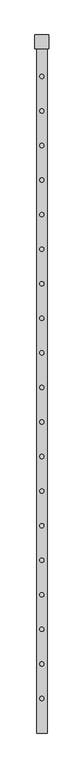
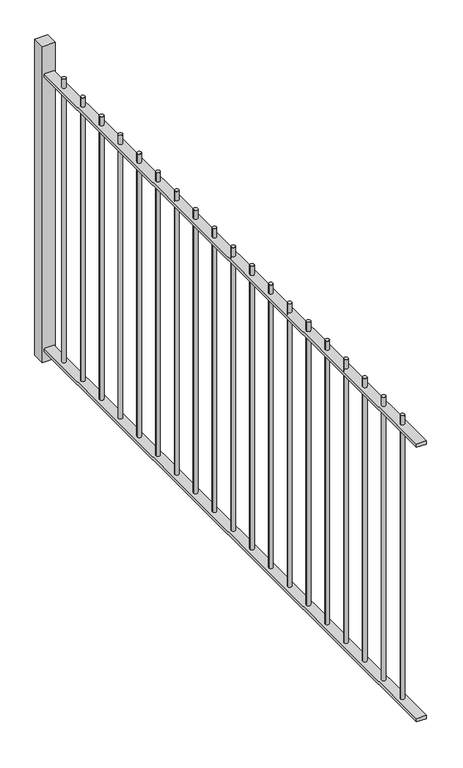
"""IFC4 building model written with IfcOpenShell, lengths in millimetres: railing geometry."""

from ifc_helpers import new_model, si_unit, point, frame, frame_2d, origin, place, context, project, spatial, polyline, circle_curve, trimmed, segment, composite_curve, outline, extrude, source, transform, mapped, element, save


def railing_93278f43(model_context):
    return source(origin(), model_context, "Body", "SweptSolid", [
        extrude(outline(polyline([(-6549.419961, -691.1119119), (-6489.419961, -691.1119119), (-6489.419961, -4691.1119119), (-6549.419961, -4691.1119119), (-6549.419961, -691.1119119)])), frame((0.0, 0.0, -30.0), z_axis=(0.0, 0.0, 1.0), x_axis=(1.0, 0.0, 0.0)), (0.0, 0.0, 1.0), 20.0),
        extrude(outline(polyline([(-6549.419961, -691.1119119), (-6489.419961, -691.1119119), (-6489.419961, -4691.1119119), (-6549.419961, -4691.1119119), (-6549.419961, -691.1119119)])), frame((0.0, 0.0, 1750.0), z_axis=(0.0, 0.0, 1.0), x_axis=(1.0, 0.0, 0.0)), (0.0, 0.0, 1.0), 20.0),
        extrude(outline(composite_curve([segment(trimmed(circle_curve(frame_2d((-6519.419961, -4491.1119119)), 12.5), [point((-6531.919961, -4491.1119119))], [point((-6506.919961, -4491.1119119))], False, "CARTESIAN"), True, "CONTINUOUS"), segment(trimmed(circle_curve(frame_2d((-6519.419961, -4491.1119119)), 12.5), [point((-6506.919961, -4491.1119119))], [point((-6531.919961, -4491.1119119))], False, "CARTESIAN"), True, "CONTINUOUS")], self_intersect=False)), frame((0.0, 0.0, -10.0), z_axis=(0.0, 0.0, 1.0), x_axis=(1.0, 0.0, 0.0)), (0.0, 0.0, 1.0), 1840.0),
        extrude(outline(composite_curve([segment(trimmed(circle_curve(frame_2d((-6519.419961, -4291.1119119)), 12.5), [point((-6531.919961, -4291.1119119))], [point((-6506.919961, -4291.1119119))], False, "CARTESIAN"), True, "CONTINUOUS"), segment(trimmed(circle_curve(frame_2d((-6519.419961, -4291.1119119)), 12.5), [point((-6506.919961, -4291.1119119))], [point((-6531.919961, -4291.1119119))], False, "CARTESIAN"), True, "CONTINUOUS")], self_intersect=False)), frame((0.0, 0.0, -10.0), z_axis=(0.0, 0.0, 1.0), x_axis=(1.0, 0.0, 0.0)), (0.0, 0.0, 1.0), 1840.0),
        extrude(outline(composite_curve([segment(trimmed(circle_curve(frame_2d((-6519.419961, -4091.1119119)), 12.5), [point((-6531.919961, -4091.1119119))], [point((-6506.919961, -4091.1119119))], False, "CARTESIAN"), True, "CONTINUOUS"), segment(trimmed(circle_curve(frame_2d((-6519.419961, -4091.1119119)), 12.5), [point((-6506.919961, -4091.1119119))], [point((-6531.919961, -4091.1119119))], False, "CARTESIAN"), True, "CONTINUOUS")], self_intersect=False)), frame((0.0, 0.0, -10.0), z_axis=(0.0, 0.0, 1.0), x_axis=(1.0, 0.0, 0.0)), (0.0, 0.0, 1.0), 1840.0),
        extrude(outline(composite_curve([segment(trimmed(circle_curve(frame_2d((-6519.419961, -3891.1119119)), 12.5), [point((-6531.919961, -3891.1119119))], [point((-6506.919961, -3891.1119119))], False, "CARTESIAN"), True, "CONTINUOUS"), segment(trimmed(circle_curve(frame_2d((-6519.419961, -3891.1119119)), 12.5), [point((-6506.919961, -3891.1119119))], [point((-6531.919961, -3891.1119119))], False, "CARTESIAN"), True, "CONTINUOUS")], self_intersect=False)), frame((0.0, 0.0, -10.0), z_axis=(0.0, 0.0, 1.0), x_axis=(1.0, 0.0, 0.0)), (0.0, 0.0, 1.0), 1840.0),
        extrude(outline(composite_curve([segment(trimmed(circle_curve(frame_2d((-6519.419961, -3691.1119119)), 12.5), [point((-6531.919961, -3691.1119119))], [point((-6506.919961, -3691.1119119))], False, "CARTESIAN"), True, "CONTINUOUS"), segment(trimmed(circle_curve(frame_2d((-6519.419961, -3691.1119119)), 12.5), [point((-6506.919961, -3691.1119119))], [point((-6531.919961, -3691.1119119))], False, "CARTESIAN"), True, "CONTINUOUS")], self_intersect=False)), frame((0.0, 0.0, -10.0), z_axis=(0.0, 0.0, 1.0), x_axis=(1.0, 0.0, 0.0)), (0.0, 0.0, 1.0), 1840.0),
        extrude(outline(composite_curve([segment(trimmed(circle_curve(frame_2d((-6519.419961, -3491.1119119)), 12.5), [point((-6531.919961, -3491.1119119))], [point((-6506.919961, -3491.1119119))], False, "CARTESIAN"), True, "CONTINUOUS"), segment(trimmed(circle_curve(frame_2d((-6519.419961, -3491.1119119)), 12.5), [point((-6506.919961, -3491.1119119))], [point((-6531.919961, -3491.1119119))], False, "CARTESIAN"), True, "CONTINUOUS")], self_intersect=False)), frame((0.0, 0.0, -10.0), z_axis=(0.0, 0.0, 1.0), x_axis=(1.0, 0.0, 0.0)), (0.0, 0.0, 1.0), 1840.0),
        extrude(outline(composite_curve([segment(trimmed(circle_curve(frame_2d((-6519.419961, -3291.1119119)), 12.5), [point((-6531.919961, -3291.1119119))], [point((-6506.919961, -3291.1119119))], False, "CARTESIAN"), True, "CONTINUOUS"), segment(trimmed(circle_curve(frame_2d((-6519.419961, -3291.1119119)), 12.5), [point((-6506.919961, -3291.1119119))], [point((-6531.919961, -3291.1119119))], False, "CARTESIAN"), True, "CONTINUOUS")], self_intersect=False)), frame((0.0, 0.0, -10.0), z_axis=(0.0, 0.0, 1.0), x_axis=(1.0, 0.0, 0.0)), (0.0, 0.0, 1.0), 1840.0),
        extrude(outline(composite_curve([segment(trimmed(circle_curve(frame_2d((-6519.419961, -3091.1119119)), 12.5), [point((-6531.919961, -3091.1119119))], [point((-6506.919961, -3091.1119119))], False, "CARTESIAN"), True, "CONTINUOUS"), segment(trimmed(circle_curve(frame_2d((-6519.419961, -3091.1119119)), 12.5), [point((-6506.919961, -3091.1119119))], [point((-6531.919961, -3091.1119119))], False, "CARTESIAN"), True, "CONTINUOUS")], self_intersect=False)), frame((0.0, 0.0, -10.0), z_axis=(0.0, 0.0, 1.0), x_axis=(1.0, 0.0, 0.0)), (0.0, 0.0, 1.0), 1840.0),
        extrude(outline(composite_curve([segment(trimmed(circle_curve(frame_2d((-6519.419961, -2891.1119119)), 12.5), [point((-6531.919961, -2891.1119119))], [point((-6506.919961, -2891.1119119))], False, "CARTESIAN"), True, "CONTINUOUS"), segment(trimmed(circle_curve(frame_2d((-6519.419961, -2891.1119119)), 12.5), [point((-6506.919961, -2891.1119119))], [point((-6531.919961, -2891.1119119))], False, "CARTESIAN"), True, "CONTINUOUS")], self_intersect=False)), frame((0.0, 0.0, -10.0), z_axis=(0.0, 0.0, 1.0), x_axis=(1.0, 0.0, 0.0)), (0.0, 0.0, 1.0), 1840.0),
        extrude(outline(composite_curve([segment(trimmed(circle_curve(frame_2d((-6519.419961, -2691.1119119)), 12.5), [point((-6531.919961, -2691.1119119))], [point((-6506.919961, -2691.1119119))], False, "CARTESIAN"), True, "CONTINUOUS"), segment(trimmed(circle_curve(frame_2d((-6519.419961, -2691.1119119)), 12.5), [point((-6506.919961, -2691.1119119))], [point((-6531.919961, -2691.1119119))], False, "CARTESIAN"), True, "CONTINUOUS")], self_intersect=False)), frame((0.0, 0.0, -10.0), z_axis=(0.0, 0.0, 1.0), x_axis=(1.0, 0.0, 0.0)), (0.0, 0.0, 1.0), 1840.0),
        extrude(outline(composite_curve([segment(trimmed(circle_curve(frame_2d((-6519.419961, -2491.1119119)), 12.5), [point((-6531.919961, -2491.1119119))], [point((-6506.919961, -2491.1119119))], False, "CARTESIAN"), True, "CONTINUOUS"), segment(trimmed(circle_curve(frame_2d((-6519.419961, -2491.1119119)), 12.5), [point((-6506.919961, -2491.1119119))], [point((-6531.919961, -2491.1119119))], False, "CARTESIAN"), True, "CONTINUOUS")], self_intersect=False)), frame((0.0, 0.0, -10.0), z_axis=(0.0, 0.0, 1.0), x_axis=(1.0, 0.0, 0.0)), (0.0, 0.0, 1.0), 1840.0),
        extrude(outline(composite_curve([segment(trimmed(circle_curve(frame_2d((-6519.419961, -2291.1119119)), 12.5), [point((-6531.919961, -2291.1119119))], [point((-6506.919961, -2291.1119119))], False, "CARTESIAN"), True, "CONTINUOUS"), segment(trimmed(circle_curve(frame_2d((-6519.419961, -2291.1119119)), 12.5), [point((-6506.919961, -2291.1119119))], [point((-6531.919961, -2291.1119119))], False, "CARTESIAN"), True, "CONTINUOUS")], self_intersect=False)), frame((0.0, 0.0, -10.0), z_axis=(0.0, 0.0, 1.0), x_axis=(1.0, 0.0, 0.0)), (0.0, 0.0, 1.0), 1840.0),
        extrude(outline(composite_curve([segment(trimmed(circle_curve(frame_2d((-6519.419961, -2091.1119119)), 12.5), [point((-6531.919961, -2091.1119119))], [point((-6506.919961, -2091.1119119))], False, "CARTESIAN"), True, "CONTINUOUS"), segment(trimmed(circle_curve(frame_2d((-6519.419961, -2091.1119119)), 12.5), [point((-6506.919961, -2091.1119119))], [point((-6531.919961, -2091.1119119))], False, "CARTESIAN"), True, "CONTINUOUS")], self_intersect=False)), frame((0.0, 0.0, -10.0), z_axis=(0.0, 0.0, 1.0), x_axis=(1.0, 0.0, 0.0)), (0.0, 0.0, 1.0), 1840.0),
        extrude(outline(composite_curve([segment(trimmed(circle_curve(frame_2d((-6519.419961, -1891.1119119)), 12.5), [point((-6531.919961, -1891.1119119))], [point((-6506.919961, -1891.1119119))], False, "CARTESIAN"), True, "CONTINUOUS"), segment(trimmed(circle_curve(frame_2d((-6519.419961, -1891.1119119)), 12.5), [point((-6506.919961, -1891.1119119))], [point((-6531.919961, -1891.1119119))], False, "CARTESIAN"), True, "CONTINUOUS")], self_intersect=False)), frame((0.0, 0.0, -10.0), z_axis=(0.0, 0.0, 1.0), x_axis=(1.0, 0.0, 0.0)), (0.0, 0.0, 1.0), 1840.0),
        extrude(outline(composite_curve([segment(trimmed(circle_curve(frame_2d((-6519.419961, -1691.1119119)), 12.5), [point((-6531.919961, -1691.1119119))], [point((-6506.919961, -1691.1119119))], False, "CARTESIAN"), True, "CONTINUOUS"), segment(trimmed(circle_curve(frame_2d((-6519.419961, -1691.1119119)), 12.5), [point((-6506.919961, -1691.1119119))], [point((-6531.919961, -1691.1119119))], False, "CARTESIAN"), True, "CONTINUOUS")], self_intersect=False)), frame((0.0, 0.0, -10.0), z_axis=(0.0, 0.0, 1.0), x_axis=(1.0, 0.0, 0.0)), (0.0, 0.0, 1.0), 1840.0),
        extrude(outline(composite_curve([segment(trimmed(circle_curve(frame_2d((-6519.419961, -1491.1119119)), 12.5), [point((-6531.919961, -1491.1119119))], [point((-6506.919961, -1491.1119119))], False, "CARTESIAN"), True, "CONTINUOUS"), segment(trimmed(circle_curve(frame_2d((-6519.419961, -1491.1119119)), 12.5), [point((-6506.919961, -1491.1119119))], [point((-6531.919961, -1491.1119119))], False, "CARTESIAN"), True, "CONTINUOUS")], self_intersect=False)), frame((0.0, 0.0, -10.0), z_axis=(0.0, 0.0, 1.0), x_axis=(1.0, 0.0, 0.0)), (0.0, 0.0, 1.0), 1840.0),
        extrude(outline(composite_curve([segment(trimmed(circle_curve(frame_2d((-6519.419961, -1291.1119119)), 12.5), [point((-6531.919961, -1291.1119119))], [point((-6506.919961, -1291.1119119))], False, "CARTESIAN"), True, "CONTINUOUS"), segment(trimmed(circle_curve(frame_2d((-6519.419961, -1291.1119119)), 12.5), [point((-6506.919961, -1291.1119119))], [point((-6531.919961, -1291.1119119))], False, "CARTESIAN"), True, "CONTINUOUS")], self_intersect=False)), frame((0.0, 0.0, -10.0), z_axis=(0.0, 0.0, 1.0), x_axis=(1.0, 0.0, 0.0)), (0.0, 0.0, 1.0), 1840.0),
        extrude(outline(composite_curve([segment(trimmed(circle_curve(frame_2d((-6519.419961, -1091.1119119)), 12.5), [point((-6531.919961, -1091.1119119))], [point((-6506.919961, -1091.1119119))], False, "CARTESIAN"), True, "CONTINUOUS"), segment(trimmed(circle_curve(frame_2d((-6519.419961, -1091.1119119)), 12.5), [point((-6506.919961, -1091.1119119))], [point((-6531.919961, -1091.1119119))], False, "CARTESIAN"), True, "CONTINUOUS")], self_intersect=False)), frame((0.0, 0.0, -10.0), z_axis=(0.0, 0.0, 1.0), x_axis=(1.0, 0.0, 0.0)), (0.0, 0.0, 1.0), 1840.0),
        extrude(outline(composite_curve([segment(trimmed(circle_curve(frame_2d((-6519.419961, -891.1119119)), 12.5), [point((-6531.919961, -891.1119119))], [point((-6506.919961, -891.1119119))], False, "CARTESIAN"), True, "CONTINUOUS"), segment(trimmed(circle_curve(frame_2d((-6519.419961, -891.1119119)), 12.5), [point((-6506.919961, -891.1119119))], [point((-6531.919961, -891.1119119))], False, "CARTESIAN"), True, "CONTINUOUS")], self_intersect=False)), frame((0.0, 0.0, -10.0), z_axis=(0.0, 0.0, 1.0), x_axis=(1.0, 0.0, 0.0)), (0.0, 0.0, 1.0), 1840.0),
        extrude(outline(polyline([(-6479.419961, -651.1119119), (-6479.419961, -731.1119119), (-6559.419961, -731.1119119), (-6559.419961, -651.1119119), (-6479.419961, -651.1119119)])), frame((0.0, 0.0, -100.0), z_axis=(0.0, 0.0, 1.0), x_axis=(1.0, 0.0, 0.0)), (0.0, 0.0, 1.0), 2050.0),
    ])


if __name__ == "__main__":
    model = new_model("IFC4")
    model_context = context("Model", 3, world=origin())
    ifc_project = project(units=[si_unit("LENGTHUNIT", "METRE", prefix="MILLI")], contexts=[model_context])
    site = spatial("IfcSite", under=ifc_project)
    building = spatial("IfcBuilding", under=site)
    placement = place(None, origin())
    railing_shape = railing_93278f43(model_context)
    element("IfcRailing", 1, at=placement, inside=building, context=model_context, shape_type="MappedRepresentation", body=[
        mapped(railing_shape, transform((0.0, 0.0, 0.0), x_axis=(1.0, 0.0, 0.0), y_axis=(0.0, 1.0, 0.0), z_axis=(0.0, 0.0, 1.0))),
    ])
    save(model, "model.ifc")

# Revit data of these elements
# Element 1 (IfcRailing)
#   Materials on its faces: "NLRS_h2_staal_generiek zwart_gen_rsf", "NLRS_h2_staal_gen_rsf"
# Materials
#   "NLRS_h2_staal_generiek zwart_gen_rsf": class "Metal", colour RGB 189 187 185, transparency 0, Manufacturer = "RevitGG", URL = "www.revitgg.nl", Description = "Staal, generiek materiaal", Cost = 0
#   "NLRS_h2_staal_gen_rsf": class "H - Metaal", colour RGB 189 187 185, transparency 0, Keynote = "h2", Model = "generiek", Manufacturer = "Revit Standards Foundation", URL = "www.revitstandards.org", Description = "staal", Cost = 0
